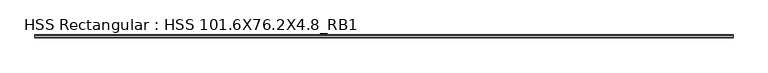
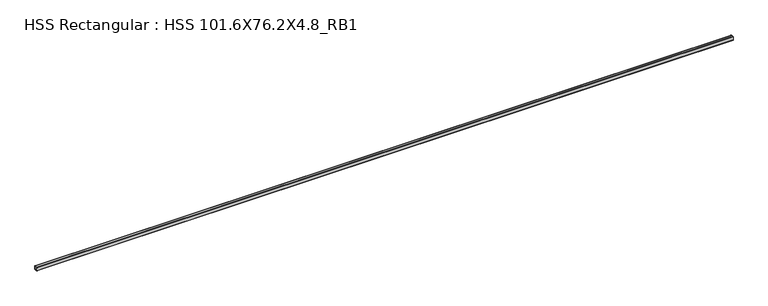
"""IFC4 building model written with IfcOpenShell, lengths in millimetres: beam geometry, HSS Rectangular : HSS 101.6X76.2X4.8_RB1."""

import ifcopenshell
import ifcopenshell.guid

model = None  # the IFC model being written
_history = None  # IfcOwnerHistory: only IFC2X3 demands one
_inside = {}  # id of a spatial element -> (the spatial element, [elements in it])
_under = {}  # id of a project, library or spatial element -> (it, [spatial elements below it])
_declared = {}  # id of a project -> (the project, [libraries it declares])
_typed = {}  # id of a type object -> (the type object, [elements of that type])
_made_of = {}  # id of a material, layer set ... -> (it, [elements and type objects made of it])


def new_model(schema):
    """Start an empty IFC model of exactly this schema.

    Asked for "IFC4X3", IfcOpenShell would pick the latest addendum, in which some entities
    have other attributes; the version numbers below select the first issue.
    IFC2X3 requires an IfcOwnerHistory on every rooted entity: one is made here for all.
    """
    global model, _history
    if schema == "IFC4X3":
        model = ifcopenshell.file(schema_version=(4, 3, 0, 0))
    else:
        model = ifcopenshell.file(schema=schema)
    _inside.clear()
    _under.clear()
    _declared.clear()
    _typed.clear()
    _made_of.clear()
    _history = None
    if model.schema == "IFC2X3":
        org = make("IfcOrganization", Name="unknown")
        user = make(
            "IfcPersonAndOrganization",
            ThePerson=make("IfcPerson", FamilyName="unknown"),
            TheOrganization=org,
        )
        app = make(
            "IfcApplication",
            ApplicationDeveloper=org,
            Version="unknown",
            ApplicationFullName="unknown",
            ApplicationIdentifier="unknown",
        )
        _history = make(
            "IfcOwnerHistory",
            OwningUser=user,
            OwningApplication=app,
            ChangeAction="ADDED",
            CreationDate=0,
        )
    return model


def make(cls, **values):
    """One entity of the class cls with the attributes given. An attribute that is None is left unset."""
    return model.create_entity(
        cls, **{name: value for name, value in values.items() if value is not None}
    )


def rooted(cls, **values):
    """An entity with a GlobalId (a new one), such as an element, a storey or a relation."""
    return make(cls, GlobalId=ifcopenshell.guid.new(), OwnerHistory=_history, **values)


def si_unit(unit_type, name, prefix=None):
    """IfcSIUnit, for example si_unit("LENGTHUNIT", "METRE", prefix="MILLI")."""
    return make("IfcSIUnit", UnitType=unit_type, Prefix=prefix, Name=name)


def assignment(units):
    """IfcUnitAssignment: the units of a project."""
    return None if units is None else make("IfcUnitAssignment", Units=units)


def point(xyz):
    """IfcCartesianPoint."""
    return None if xyz is None else make("IfcCartesianPoint", Coordinates=xyz)


def direction(xyz):
    """IfcDirection."""
    return None if xyz is None else make("IfcDirection", DirectionRatios=xyz)


def frame(location, z_axis=None, x_axis=None):
    """IfcAxis2Placement3D, a coordinate frame: its origin and axes. An axis left out is left unset."""
    return make(
        "IfcAxis2Placement3D",
        Location=point(location),
        Axis=direction(z_axis),
        RefDirection=direction(x_axis),
    )


def frame_2d(location, x_axis=None):
    """IfcAxis2Placement2D, a coordinate frame in the plane: its origin and x axis."""
    return make(
        "IfcAxis2Placement2D", Location=point(location), RefDirection=direction(x_axis)
    )


def origin():
    """The frame at (0, 0, 0) with its axes left unset."""
    return frame((0.0, 0.0, 0.0))


def place(relative_to, where):
    """IfcLocalPlacement: puts the frame where relative to a parent placement (None: the world)."""
    return make(
        "IfcLocalPlacement", PlacementRelTo=relative_to, RelativePlacement=where
    )


def context(
    kind, dimensions, precision=None, world=None, true_north=None, identifier=None
):
    """IfcGeometricRepresentationContext, for example the 3D "Model" context."""
    return make(
        "IfcGeometricRepresentationContext",
        ContextIdentifier=identifier,
        ContextType=kind,
        CoordinateSpaceDimension=dimensions,
        Precision=precision,
        WorldCoordinateSystem=world,
        TrueNorth=true_north,
    )


def project(units=None, contexts=None):
    """IfcProject with its units and contexts."""
    return rooted(
        "IfcProject",
        Name="project",
        RepresentationContexts=contexts,
        UnitsInContext=assignment(units),
    )


def spatial(cls, under=None, at=None, **own):
    """A site, building, storey or space (cls), placed at a placement, below another one or the project."""
    s = rooted(cls, ObjectPlacement=at, **own)
    if under is not None:
        _under.setdefault(under.id(), (under, []))[1].append(s)
    return s


def polyline(points):
    """IfcPolyline through the points."""
    return make("IfcPolyline", Points=[point(p) for p in points])


def circle_curve(where, radius):
    """IfcCircle in the frame where."""
    return make("IfcCircle", Position=where, Radius=radius)


def trimmed(basis, trim1, trim2, sense, master):
    """IfcTrimmedCurve: the piece of a basis curve between two trims."""
    return make(
        "IfcTrimmedCurve",
        BasisCurve=basis,
        Trim1=trim1,
        Trim2=trim2,
        SenseAgreement=sense,
        MasterRepresentation=master,
    )


def segment(curve, same_sense, transition):
    """IfcCompositeCurveSegment."""
    return make(
        "IfcCompositeCurveSegment",
        Transition=transition,
        SameSense=same_sense,
        ParentCurve=curve,
    )


def composite_curve(segments, self_intersect=None):
    """IfcCompositeCurve: segments joined end to end."""
    return make("IfcCompositeCurve", Segments=segments, SelfIntersect=self_intersect)


def outline(outer, holes=None, kind="AREA"):
    """IfcArbitraryClosedProfileDef: a profile drawn as a closed curve; with holes, ...WithVoids."""
    if holes is None:
        return make("IfcArbitraryClosedProfileDef", ProfileType=kind, OuterCurve=outer)
    return make(
        "IfcArbitraryProfileDefWithVoids",
        ProfileType=kind,
        OuterCurve=outer,
        InnerCurves=holes,
    )


def extrude(swept, where, along, depth):
    """IfcExtrudedAreaSolid: the profile swept, set in the frame where, extruded along a direction by depth."""
    return make(
        "IfcExtrudedAreaSolid",
        SweptArea=swept,
        Position=where,
        ExtrudedDirection=direction(along),
        Depth=depth,
    )


def shape(context_of_items, identifier, shape_type, items):
    """IfcShapeRepresentation: the items that make up one representation, for example the "Body"."""
    return make(
        "IfcShapeRepresentation",
        ContextOfItems=context_of_items,
        RepresentationIdentifier=identifier,
        RepresentationType=shape_type,
        Items=items,
    )


def source(mapping_origin, context_of_items, identifier, shape_type, items):
    """IfcRepresentationMap: a shape defined once, which mapped items show again and again."""
    return make(
        "IfcRepresentationMap",
        MappingOrigin=mapping_origin,
        MappedRepresentation=shape(context_of_items, identifier, shape_type, items),
    )


def transform(
    local_origin,
    x_axis=None,
    y_axis=None,
    z_axis=None,
    scale=None,
    scale2=None,
    scale3=None,
    uniform=True,
):
    """IfcCartesianTransformationOperator3D, or its non-uniform kind. x_axis, y_axis, z_axis: its Axis1, 2, 3."""
    if uniform:
        return make(
            "IfcCartesianTransformationOperator3D",
            Axis1=direction(x_axis),
            Axis2=direction(y_axis),
            LocalOrigin=point(local_origin),
            Scale=scale,
            Axis3=direction(z_axis),
        )
    return make(
        "IfcCartesianTransformationOperator3DnonUniform",
        Axis1=direction(x_axis),
        Axis2=direction(y_axis),
        LocalOrigin=point(local_origin),
        Scale=scale,
        Axis3=direction(z_axis),
        Scale2=scale2,
        Scale3=scale3,
    )


def mapped(mapping_source, mapping_target):
    """IfcMappedItem: shows the shape of a source again, moved by a transform."""
    return make(
        "IfcMappedItem", MappingSource=mapping_source, MappingTarget=mapping_target
    )


def made_of(thing, what):
    """Note that an element or type object is made of a material, layer set ...; save() writes the relation."""
    if what is not None:
        _made_of.setdefault(what.id(), (what, []))[1].append(thing)
    return thing


def element(
    cls,
    number,
    at=None,
    inside=None,
    cuts=None,
    type_object=None,
    material=None,
    context=None,
    identifier="Body",
    shape_type=None,
    held_by="IfcProductDefinitionShape",
    body=None,
    shapes=None,
    **own,
):
    """One element of the class cls, such as IfcWall. Its Tag is "e" and its number.

    at: its placement. inside: the storey or other place that contains it. cuts: it is an
    opening in that element (IfcRelVoidsElement). A single representation is given by context,
    identifier, shape_type and body (its items); several are given by shapes. held_by: the class
    of the entity that holds the representations. save() writes the other relations.
    """
    e = rooted(cls, Tag="e%d" % number, ObjectPlacement=at, **own)
    if body is not None:
        shapes = [shape(context, identifier, shape_type, body)]
    if shapes is not None:
        e.Representation = make(held_by, Representations=shapes)
    if inside is not None:
        _inside.setdefault(inside.id(), (inside, []))[1].append(e)
    if cuts is not None:
        rooted(
            "IfcRelVoidsElement", RelatingBuildingElement=cuts, RelatedOpeningElement=e
        )
    if type_object is not None:
        _typed.setdefault(type_object.id(), (type_object, []))[1].append(e)
    return made_of(e, material)


def aggregate(whole, parts):
    """IfcRelAggregates: a whole, such as a stair, and the parts it consists of."""
    return rooted("IfcRelAggregates", RelatingObject=whole, RelatedObjects=parts)


def save(model, path):
    """Write the relations noted so far, then the file.

    IfcRelAggregates (storeys below a building ...), IfcRelContainedInSpatialStructure (elements
    in a storey), IfcRelDefinesByType, IfcRelAssociatesMaterial and IfcRelDeclares: one each for
    every whole, place, type object, material and project.
    """
    for whole, parts in _under.values():
        aggregate(whole, parts)
    for where, things in _inside.values():
        rooted(
            "IfcRelContainedInSpatialStructure",
            RelatedElements=things,
            RelatingStructure=where,
        )
    for kind, things in _typed.values():
        rooted("IfcRelDefinesByType", RelatedObjects=things, RelatingType=kind)
    for what, things in _made_of.values():
        rooted("IfcRelAssociatesMaterial", RelatedObjects=things, RelatingMaterial=what)
    for by, libraries in _declared.values():
        rooted("IfcRelDeclares", RelatingContext=by, RelatedDefinitions=libraries)
    model.write(path)


def hss_rectangular_hss_101_6x76_2x4_8_rb1_8939e418(model_context):
    return source(origin(), model_context, "Body", "SweptSolid", [
        extrude(outline(composite_curve([segment(trimmed(circle_curve(frame_2d((-28.575, 41.275)), 9.525), [point((-38.1, 41.275))], [point((-28.575, 50.8))], False, "CARTESIAN"), True, "CONTINUOUS"), segment(polyline([(-28.575, 50.8), (28.575, 50.8)]), True, "CONTINUOUS"), segment(trimmed(circle_curve(frame_2d((28.575, 41.275)), 9.525), [point((28.575, 50.8))], [point((38.1, 41.275))], False, "CARTESIAN"), True, "CONTINUOUS"), segment(polyline([(38.1, 41.275), (38.1, -41.275)]), True, "CONTINUOUS"), segment(trimmed(circle_curve(frame_2d((28.575, -41.275)), 9.525), [point((38.1, -41.275))], [point((28.575, -50.8))], False, "CARTESIAN"), True, "CONTINUOUS"), segment(polyline([(28.575, -50.8), (-28.575, -50.8)]), True, "CONTINUOUS"), segment(trimmed(circle_curve(frame_2d((-28.575, -41.275)), 9.525), [point((-28.575, -50.8))], [point((-38.1, -41.275))], False, "CARTESIAN"), True, "CONTINUOUS"), segment(polyline([(-38.1, -41.275), (-38.1, 41.275)]), True, "CONTINUOUS")], self_intersect=False), holes=[composite_curve([segment(polyline([(28.575, 46.0375), (-28.575, 46.0375)]), True, "CONTINUOUS"), segment(trimmed(circle_curve(frame_2d((-28.575, 41.275)), 4.7625), [point((-28.575, 46.0375))], [point((-33.3375, 41.275))], True, "CARTESIAN"), True, "CONTINUOUS"), segment(polyline([(-33.3375, 41.275), (-33.3375, -41.275)]), True, "CONTINUOUS"), segment(trimmed(circle_curve(frame_2d((-28.575, -41.275)), 4.7625), [point((-33.3375, -41.275))], [point((-28.575, -46.0375))], True, "CARTESIAN"), True, "CONTINUOUS"), segment(polyline([(-28.575, -46.0375), (28.575, -46.0375)]), True, "CONTINUOUS"), segment(trimmed(circle_curve(frame_2d((28.575, -41.275)), 4.7625), [point((28.575, -46.0375))], [point((33.3375, -41.275))], True, "CARTESIAN"), True, "CONTINUOUS"), segment(polyline([(33.3375, -41.275), (33.3375, 41.275)]), True, "CONTINUOUS"), segment(trimmed(circle_curve(frame_2d((28.575, 41.275)), 4.7625), [point((33.3375, 41.275))], [point((28.575, 46.0375))], True, "CARTESIAN"), True, "CONTINUOUS")], self_intersect=False)]), frame((-7489.089, 0.0, 0.0), z_axis=(1.0, 0.0, 0.0), x_axis=(0.0, 1.0, 0.0)), (0.0, 0.0, 1.0), 17962.1015),
    ])


if __name__ == "__main__":
    model = new_model("IFC4")
    model_context = context("Model", 3, world=origin())
    ifc_project = project(units=[si_unit("LENGTHUNIT", "METRE", prefix="MILLI")], contexts=[model_context])
    site = spatial("IfcSite", under=ifc_project)
    building = spatial("IfcBuilding", under=site)
    placement = place(None, origin())
    hss_rectangular_hss_101_6x76_2x4_8_rb1_shape = hss_rectangular_hss_101_6x76_2x4_8_rb1_8939e418(model_context)
    element("IfcBeam", 1, ObjectType="HSS Rectangular : HSS 101.6X76.2X4.8_RB1", at=placement, inside=building, context=model_context, shape_type="MappedRepresentation", body=[
        mapped(hss_rectangular_hss_101_6x76_2x4_8_rb1_shape, transform((0.0, 0.0, 0.0), x_axis=(1.0, 0.0, 0.0), y_axis=(0.0, 1.0, 0.0), z_axis=(0.0, 0.0, 1.0))),
    ])
    save(model, "model.ifc")

# Revit data of these elements
# Type "HSS Rectangular : HSS 101.6X76.2X4.8_RB1"
#   Section Name Key = "HSS 4X3X3/16"
#   Assembly Code = "B10"
#   Width = 7.62 cm
#   Wall Nominal Thickness = 0.4763 cm
#   Wall Design Thickness = 0.442 cm
#   Torsional Moment of Inertia = 260.561 cm⁴
#   Torsional Modulus = 61.2876 cm³
#   Section Area = 14.4516 cm²
#   Plastic Modulus weak axis = 40.3122 cm³
#   Plastic Modulus strong axis = 49.1612 cm³
#   Perimeter = 0.881482 m²/m
#   Outer Fillet = 0.9525 cm
#   Nominal Weight = 12.1285 kgf/m
#   Moment of Inertia weak axis = 131.529 cm⁴
#   Moment of Inertia strong axis = 205.202 cm⁴
#   Inner Fillet = 0.4763 cm
#   Height = 10.16 cm
#   Elastic Modulus weak axis = 34.4128 cm³
#   Elastic Modulus strong axis = 40.476 cm³
#   Centroid Vertical = 5.08 cm
#   Centroid Horizontal = 3.81 cm
#   Length [instance default] = 1524 mm
#   Structural Material [instance default] = Steel ASTM A500, Grade B, Rectangular and Square
#   Principal Axes Angle = 0
# Element 1 (IfcBeam, "HSS Rectangular : HSS 101.6X76.2X4.8_RB1")
#   Structural Material = Steel ASTM A992
#   Materials on its faces: "Steel ASTM A992"
# Materials
#   "Steel ASTM A500, Grade B, Rectangular and Square": class "Metal", colour RGB 199 199 199, transparency 0, Description = "Carbon steel", Cost = 0
#   "Steel ASTM A992": class "Metal", colour RGB 199 199 199, transparency 0, Description = "Structural steel 50ksi", Cost = 0
